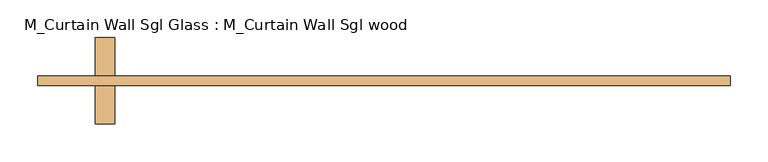
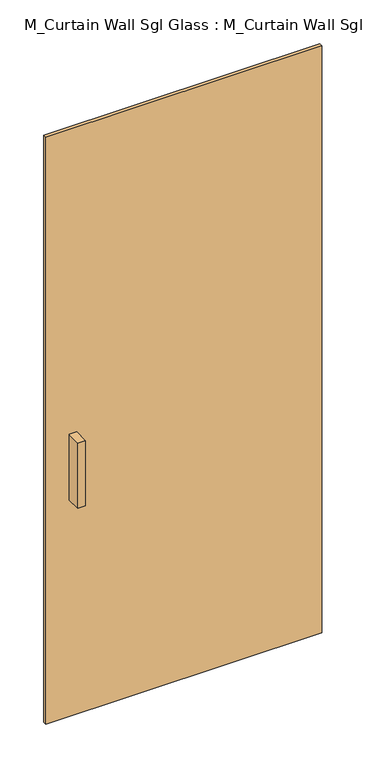
"""IFC4 building model written with IfcOpenShell, lengths in millimetres: door geometry, M_Curtain Wall Sgl Glass : M_Curtain Wall Sgl wood."""

from ifc_helpers import new_model, si_unit, frame, origin, origin_with_axes, place, context, project, spatial, polyline, outline, extrude, source, transform, mapped, element, save


def m_curtain_wall_sgl_glass_m_curtain_wall_sgl_wood_81fc5990(model_context):
    return source(origin(), model_context, "Body", "SweptSolid", [
        extrude(outline(polyline([(-356.5, 12.5), (-356.5, -38.3), (-381.9, -38.3), (-381.9, 12.5), (-356.5, 12.5)])), frame((0.0, 0.0, 762.0), z_axis=(0.0, 0.0, 1.0), x_axis=(1.0, 0.0, 0.0)), (0.0, 0.0, 1.0), 228.6),
        extrude(outline(polyline([(-381.9, -101.8), (-381.9, -51.0), (-356.5, -51.0), (-356.5, -101.8), (-381.9, -101.8)])), frame((0.0, 0.0, 762.0), z_axis=(0.0, 0.0, 1.0), x_axis=(1.0, 0.0, 0.0)), (0.0, 0.0, 1.0), 228.6),
        extrude(outline(polyline([(458.1, -51.0), (-458.1, -51.0), (-458.1, -38.3), (458.1, -38.3), (458.1, -51.0)])), origin_with_axes(), (0.0, 0.0, 1.0), 2060.0),
    ])


if __name__ == "__main__":
    model = new_model("IFC4")
    model_context = context("Model", 3, world=origin())
    ifc_project = project(units=[si_unit("LENGTHUNIT", "METRE", prefix="MILLI")], contexts=[model_context])
    site = spatial("IfcSite", under=ifc_project)
    building = spatial("IfcBuilding", under=site)
    placement = place(None, origin())
    m_curtain_wall_sgl_glass_m_curtain_wall_sgl_wood_shape = m_curtain_wall_sgl_glass_m_curtain_wall_sgl_wood_81fc5990(model_context)
    element("IfcDoor", 1, ObjectType="M_Curtain Wall Sgl Glass : M_Curtain Wall Sgl wood", at=placement, inside=building, context=model_context, shape_type="MappedRepresentation", body=[
        mapped(m_curtain_wall_sgl_glass_m_curtain_wall_sgl_wood_shape, transform((0.0, 0.0, 0.0), x_axis=(1.0, 0.0, 0.0), y_axis=(0.0, 1.0, 0.0), z_axis=(0.0, 0.0, 1.0))),
    ])
    save(model, "model.ifc")

# Revit data of these elements
# Type "M_Curtain Wall Sgl Glass : M_Curtain Wall Sgl wood"
#   Model = "12345669"
#   Manufacturer = "Dublin Doors"
#   Description = "Single Wood Door"
#   Type Mark = "45"
#   Fire Rating = "60M"
#   COBie.Type.CreatedBy = "design@eagle.com"
#   COBie.Type.CreatedOn = "2016-09-13T05:47:35"
#   COBie.Type.Name = "Doors_M_Curtain Wall Sgl Glass_M_Curtain Wall Sgl wood"
#   COBie.Type.Category = "23-30 10 00 : Doors"
#   COBie.Type.Description = "Single Wood Door"
#   COBie.Type.Manufacturer = "Dublin Doors"
#   COBie.Type.ModelNumber = "12345669"
#   Construction Type Id = "opn-d36"
#   Analytic Construction = "Wood panel"
#   COBie.Type.ReplacementCost = 0
#   Offset = 51 mm
#   Heat Transfer Coefficient (U) = 3.8042 W/(m²·K)
#   COBie.Type = yes
#   Function = 1
#   Glazing Material = Door - Panel
#   Visual Light Transmittance = 0
#   Solar Heat Gain Coefficient = 0
# Element 1 (IfcDoor, "M_Curtain Wall Sgl Glass : M_Curtain Wall Sgl wood")
#   Materials on its faces: "Aluminum", "Door - Panel"
# Materials
#   "Door - Panel": class "Wood", colour RGB 210 159 95, transparency 0
#   "Aluminum": class "Metal", colour RGB 247 247 247, transparency 0, Description = "Aluminum 6061", Cost = 0
